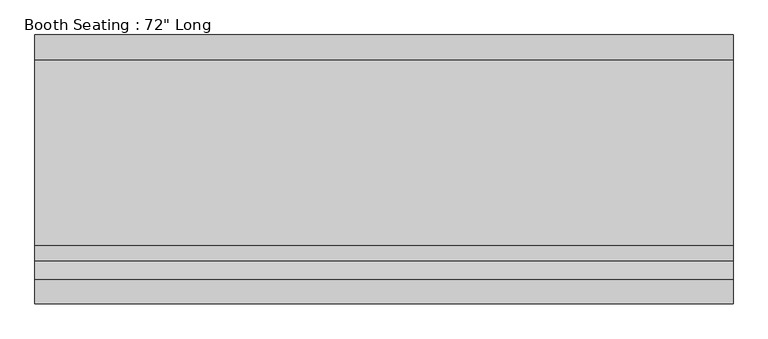
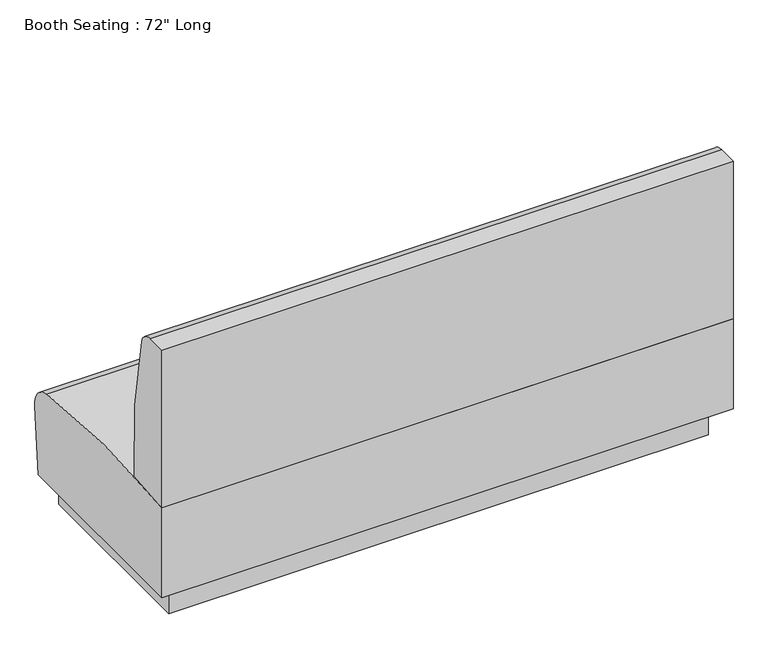
"""IFC4 building model written with IfcOpenShell, lengths in millimetres: furniture geometry."""

from ifc_helpers import new_model, si_unit, point, frame, frame_2d, origin, origin_with_axes, place, context, project, spatial, polyline, circle_curve, trimmed, segment, composite_curve, outline, extrude, source, transform, mapped, element, save


def furniture_925b8007(model_context):
    return source(origin(), model_context, "Body", "SweptSolid", [
        extrude(outline(composite_curve([segment(polyline([(-355.6, 939.8), (-292.2747753, 939.8)]), True, "CONTINUOUS"), segment(trimmed(circle_curve(frame_2d((-292.2747753, 889.0)), 50.8), [point((-292.2747753, 939.8))], [point((-242.7504703, 900.3129667))], False, "CARTESIAN"), True, "CONTINUOUS"), segment(trimmed(circle_curve(frame_2d((-1896.6191414, 522.5154157)), 1696.4706218), [point((-242.7504703, 900.3129667))], [point((-203.2, 420.809063))], False, "CARTESIAN"), True, "CONTINUOUS"), segment(polyline([(-203.2, 420.809063), (-355.6, 406.4), (-355.6, 939.8)]), True, "CONTINUOUS")], self_intersect=False)), frame((-914.4, 0.0, 0.0), z_axis=(1.0, 0.0, 0.0), x_axis=(0.0, 1.0, 0.0)), (0.0, 0.0, 1.0), 1828.8),
        extrude(outline(composite_curve([segment(polyline([(348.6009692, 322.4116302), (330.2, 101.6), (-355.6, 101.6), (-355.6, 406.4)]), True, "CONTINUOUS"), segment(trimmed(circle_curve(frame_2d((-44.6835428, -2068.9155338)), 2494.7657275), [point((-355.6, 406.4))], [point((282.6626275, 404.2808838))], False, "CARTESIAN"), True, "CONTINUOUS"), segment(trimmed(circle_curve(frame_2d((272.6641824, 328.7396957)), 76.2), [point((282.6626275, 404.2808838))], [point((348.6009692, 322.4116302))], False, "CARTESIAN"), True, "CONTINUOUS")], self_intersect=False)), frame((-914.4, 0.0, 0.0), z_axis=(1.0, 0.0, 0.0), x_axis=(0.0, 1.0, 0.0)), (0.0, 0.0, 1.0), 1828.8),
        extrude(outline(polyline([(863.6, -304.8), (-863.6, -304.8), (-863.6, 304.8), (863.6, 304.8), (863.6, -304.8)])), origin_with_axes(), (0.0, 0.0, 1.0), 101.6),
    ])


if __name__ == "__main__":
    model = new_model("IFC4")
    model_context = context("Model", 3, world=origin())
    ifc_project = project(units=[si_unit("LENGTHUNIT", "METRE", prefix="MILLI")], contexts=[model_context])
    site = spatial("IfcSite", under=ifc_project)
    building = spatial("IfcBuilding", under=site)
    placement = place(None, origin())
    furniture_shape = furniture_925b8007(model_context)
    element("IfcFurniture", 1, ObjectType="Booth Seating : 72\" Long", at=placement, inside=building, context=model_context, shape_type="MappedRepresentation", body=[
        mapped(furniture_shape, transform((0.0, 0.0, 0.0), x_axis=(1.0, 0.0, 0.0), y_axis=(0.0, 1.0, 0.0), z_axis=(0.0, 0.0, 1.0))),
    ])
    save(model, "model.ifc")

# Revit data of these elements
# Type "Booth Seating : 72\" Long"
#   Type Mark = "SB2"
#   Seat Height = 1' - 4"
#   Length = 6' - 0"
#   Depth = 2' - 4"
#   Back Height = 3' - 1"
#   Number of Persons = 3
#   Default Elevation = 0
# Element 1 (IfcFurniture, "Booth Seating : 72\" Long")
#   Materials on its faces: "Leather, Dark Brown", "Plastic, Opaque Black"
# Materials
#   "Leather, Dark Brown": class "Textile", colour RGB 57 45 39, transparency 0, Description = "Leather, dark brown", Cost = 0
#   "Plastic, Opaque Black": class "Plastic", colour RGB 5 5 5, transparency 0, Description = "Plastic, generic, opaque black", Cost = 0
